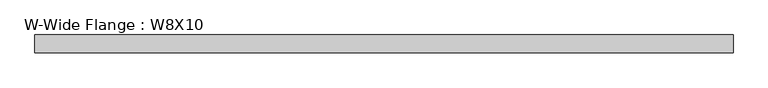
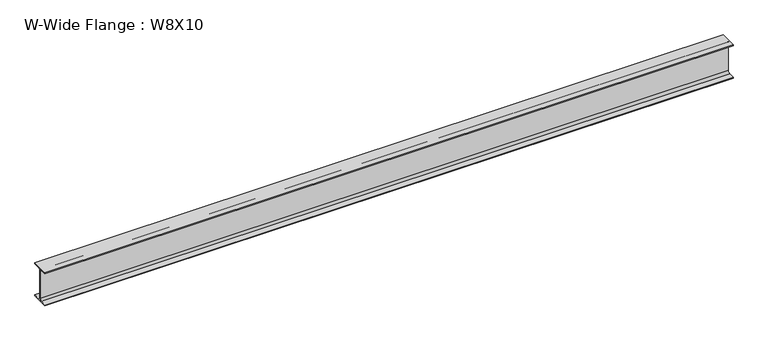
"""IFC4 building model written with IfcOpenShell, lengths in millimetres: beam geometry, W-Wide Flange : W8X10."""

from ifc_helpers import new_model, si_unit, point, frame, frame_2d, origin, place, context, project, spatial, polyline, circle_curve, trimmed, segment, composite_curve, outline, extrude, source, transform, mapped, element, save


def w_wide_flange_w8x10_be9bb2d2(model_context):
    return source(origin(), model_context, "Body", "SweptSolid", [
        extrude(outline(composite_curve([segment(polyline([(50.038, -94.996), (50.038, -100.203), (-50.038, -100.203), (-50.038, -94.996), (-14.4145, -94.996)]), True, "CONTINUOUS"), segment(trimmed(circle_curve(frame_2d((-14.4145, -82.7405)), 12.2555), [point((-14.4145, -94.996))], [point((-2.159, -82.7405))], True, "CARTESIAN"), True, "CONTINUOUS"), segment(polyline([(-2.159, -82.7405), (-2.159, 82.7405)]), True, "CONTINUOUS"), segment(trimmed(circle_curve(frame_2d((-14.4145, 82.7405)), 12.2555), [point((-2.159, 82.7405))], [point((-14.4145, 94.996))], True, "CARTESIAN"), True, "CONTINUOUS"), segment(polyline([(-14.4145, 94.996), (-50.038, 94.996), (-50.038, 100.203), (50.038, 100.203), (50.038, 94.996), (14.4145, 94.996)]), True, "CONTINUOUS"), segment(trimmed(circle_curve(frame_2d((14.4145, 82.7405)), 12.2555), [point((14.4145, 94.996))], [point((2.159, 82.7405))], True, "CARTESIAN"), True, "CONTINUOUS"), segment(polyline([(2.159, 82.7405), (2.159, -82.7405)]), True, "CONTINUOUS"), segment(trimmed(circle_curve(frame_2d((14.4145, -82.7405)), 12.2555), [point((2.159, -82.7405))], [point((14.4145, -94.996))], True, "CARTESIAN"), True, "CONTINUOUS"), segment(polyline([(14.4145, -94.996), (50.038, -94.996)]), True, "CONTINUOUS")], self_intersect=False)), frame((-2026.6421875, 0.0, 0.0), z_axis=(1.0, 0.0, 0.0), x_axis=(0.0, 1.0, 0.0)), (0.0, 0.0, 1.0), 3942.7050781),
    ])


if __name__ == "__main__":
    model = new_model("IFC4")
    model_context = context("Model", 3, world=origin())
    ifc_project = project(units=[si_unit("LENGTHUNIT", "METRE", prefix="MILLI")], contexts=[model_context])
    site = spatial("IfcSite", under=ifc_project)
    building = spatial("IfcBuilding", under=site)
    placement = place(None, origin())
    w_wide_flange_w8x10_shape = w_wide_flange_w8x10_be9bb2d2(model_context)
    element("IfcBeam", 1, ObjectType="W-Wide Flange : W8X10", at=placement, inside=building, context=model_context, shape_type="MappedRepresentation", body=[
        mapped(w_wide_flange_w8x10_shape, transform((0.0, 0.0, 0.0), x_axis=(1.0, 0.0, 0.0), y_axis=(0.0, 1.0, 0.0), z_axis=(0.0, 0.0, 1.0))),
    ])
    save(model, "model.ifc")

# Revit data of these elements
# Type "W-Wide Flange : W8X10"
#   Assembly Code = "B10"
#   W = 10
#   Length [instance default] = 1524 mm
#   bf = 100.076 mm
#   d = 200.406 mm
#   k = 17.463 mm
#   k2 = 12.255 mm
#   tf = 5.207 mm
#   tw = 4.318 mm
#   A = 0.00190967 m²
#   Structural Material [instance default] = Steel ASTM A992
# Element 1 (IfcBeam, "W-Wide Flange : W8X10")
#   Structural Material = Aluminum, Anodized Red
#   Materials on its faces: "Aluminum, Anodized Red"
# Materials
#   "Steel ASTM A992": class "Metal", colour RGB 128 0 0, transparency 0, Description = "Structural steel 50ksi", Cost = 0
#   "Aluminum, Anodized Red": class "Metal", colour RGB 120 120 120, transparency 0, Description = "Anodized aluminum, red", Cost = 0
